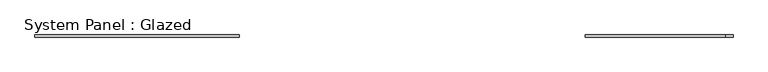
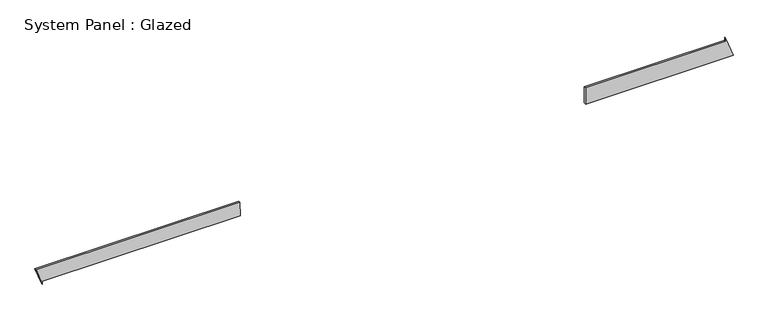
"""IFC4 building model written with IfcOpenShell, lengths in millimetres: plate geometry, System Panel : Glazed."""

from ifc_helpers import new_model, si_unit, frame, origin, place, context, project, spatial, polyline, outline, extrude, source, transform, mapped, element, save


def system_panel_glazed_c0f42e98(model_context):
    return source(origin(), model_context, "Body", "SweptSolid", [
        extrude(outline(polyline([(0.0, 2327.1115757), (0.0, 4034.6007191), (234.3998836, 3949.9537418), (199.0445445, 3949.9522175), (199.114455, 2328.4254713), (0.0, 2327.1115757)])), frame((0.0, -49.5, 0.0), z_axis=(0.0, 1.0, 0.0), x_axis=(0.0, 0.0, 1.0)), (0.0, 0.0, 1.0), 25.0),
        extrude(outline(polyline([(0.0, -3963.5189783), (35.3553391, -3963.5189783), (35.3553391, -1673.7284407), (199.2870376, -1674.5133491), (199.3887904, -4034.6007191), (0.0, -3963.5189783)])), frame((0.0, -49.5, 0.0), z_axis=(0.0, 1.0, 0.0), x_axis=(0.0, 0.0, 1.0)), (0.0, 0.0, 1.0), 25.0),
    ])


if __name__ == "__main__":
    model = new_model("IFC4")
    model_context = context("Model", 3, world=origin())
    ifc_project = project(units=[si_unit("LENGTHUNIT", "METRE", prefix="MILLI")], contexts=[model_context])
    site = spatial("IfcSite", under=ifc_project)
    building = spatial("IfcBuilding", under=site)
    placement = place(None, origin())
    system_panel_glazed_shape = system_panel_glazed_c0f42e98(model_context)
    element("IfcPlate", 1, ObjectType="System Panel : Glazed", at=placement, inside=building, context=model_context, shape_type="MappedRepresentation", body=[
        mapped(system_panel_glazed_shape, transform((0.0, 0.0, 0.0), x_axis=(1.0, 0.0, 0.0), y_axis=(0.0, 1.0, 0.0), z_axis=(0.0, 0.0, 1.0))),
    ])
    save(model, "model.ifc")

# Revit data of these elements
# Element 1 (IfcPlate, "System Panel : Glazed")
#   Materials on its faces: "Glass"
# Materials
#   "Glass": class "Glass", colour RGB 218 227 224, transparency 0.85, Description = "Soda Lime Glass", Cost = 0
